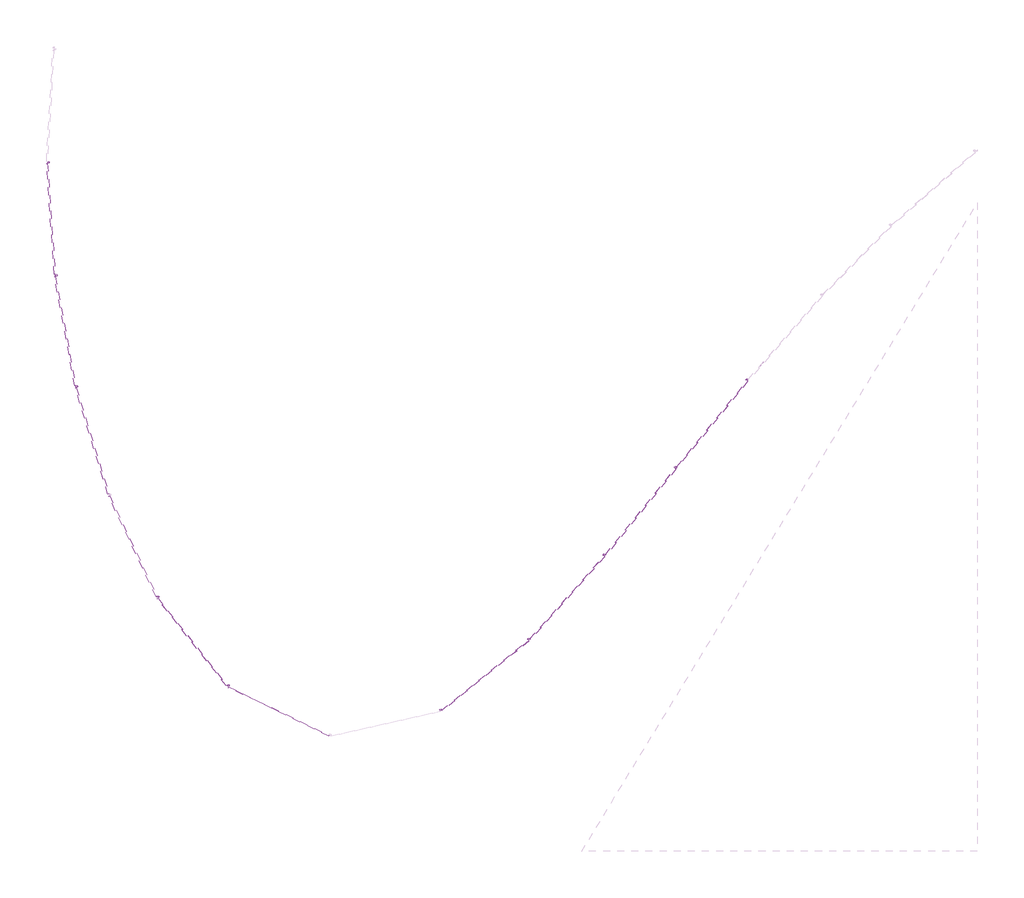
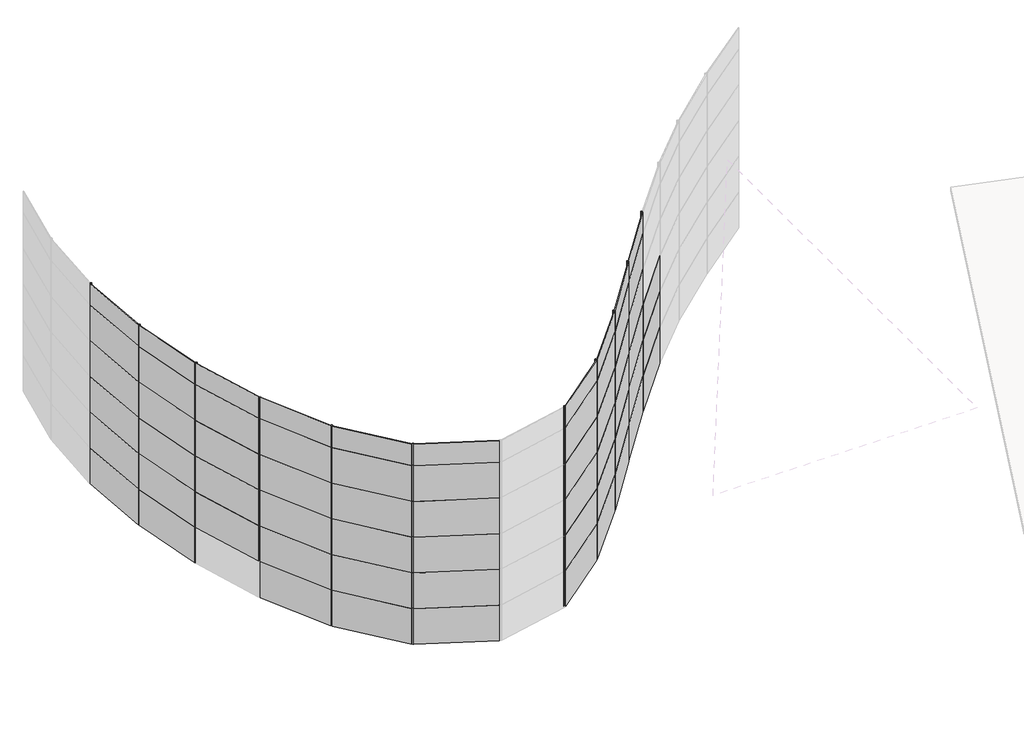
# One storey, part 4 of 8: 62 plates, 60 members.
"""IFC4 building model written with IfcOpenShell, lengths in millimetres."""

import ifcopenshell
import ifcopenshell.guid

model = None  # the IFC model being written
_history = None  # IfcOwnerHistory: only IFC2X3 demands one
_inside = {}  # id of a spatial element -> (the spatial element, [elements in it])
_under = {}  # id of a project, library or spatial element -> (it, [spatial elements below it])
_declared = {}  # id of a project -> (the project, [libraries it declares])
_typed = {}  # id of a type object -> (the type object, [elements of that type])
_made_of = {}  # id of a material, layer set ... -> (it, [elements and type objects made of it])


def new_model(schema):
    """Start an empty IFC model of exactly this schema.

    Asked for "IFC4X3", IfcOpenShell would pick the latest addendum, in which some entities
    have other attributes; the version numbers below select the first issue.
    IFC2X3 requires an IfcOwnerHistory on every rooted entity: one is made here for all.
    """
    global model, _history
    if schema == "IFC4X3":
        model = ifcopenshell.file(schema_version=(4, 3, 0, 0))
    else:
        model = ifcopenshell.file(schema=schema)
    _inside.clear()
    _under.clear()
    _declared.clear()
    _typed.clear()
    _made_of.clear()
    _history = None
    if model.schema == "IFC2X3":
        org = make("IfcOrganization", Name="unknown")
        user = make(
            "IfcPersonAndOrganization",
            ThePerson=make("IfcPerson", FamilyName="unknown"),
            TheOrganization=org,
        )
        app = make(
            "IfcApplication",
            ApplicationDeveloper=org,
            Version="unknown",
            ApplicationFullName="unknown",
            ApplicationIdentifier="unknown",
        )
        _history = make(
            "IfcOwnerHistory",
            OwningUser=user,
            OwningApplication=app,
            ChangeAction="ADDED",
            CreationDate=0,
        )
    return model


def make(cls, **values):
    """One entity of the class cls with the attributes given. An attribute that is None is left unset."""
    return model.create_entity(
        cls, **{name: value for name, value in values.items() if value is not None}
    )


def rooted(cls, **values):
    """An entity with a GlobalId (a new one), such as an element, a storey or a relation."""
    return make(cls, GlobalId=ifcopenshell.guid.new(), OwnerHistory=_history, **values)


def si_unit(unit_type, name, prefix=None):
    """IfcSIUnit, for example si_unit("LENGTHUNIT", "METRE", prefix="MILLI")."""
    return make("IfcSIUnit", UnitType=unit_type, Prefix=prefix, Name=name)


def assignment(units):
    """IfcUnitAssignment: the units of a project."""
    return None if units is None else make("IfcUnitAssignment", Units=units)


def point(xyz):
    """IfcCartesianPoint."""
    return None if xyz is None else make("IfcCartesianPoint", Coordinates=xyz)


def direction(xyz):
    """IfcDirection."""
    return None if xyz is None else make("IfcDirection", DirectionRatios=xyz)


def frame(location, z_axis=None, x_axis=None):
    """IfcAxis2Placement3D, a coordinate frame: its origin and axes. An axis left out is left unset."""
    return make(
        "IfcAxis2Placement3D",
        Location=point(location),
        Axis=direction(z_axis),
        RefDirection=direction(x_axis),
    )


def frame_2d(location, x_axis=None):
    """IfcAxis2Placement2D, a coordinate frame in the plane: its origin and x axis."""
    return make(
        "IfcAxis2Placement2D", Location=point(location), RefDirection=direction(x_axis)
    )


def origin():
    """The frame at (0, 0, 0) with its axes left unset."""
    return frame((0.0, 0.0, 0.0))


def origin_with_axes():
    """The frame at (0, 0, 0) with the z axis (0, 0, 1) and the x axis (1, 0, 0) written out."""
    return frame((0.0, 0.0, 0.0), z_axis=(0.0, 0.0, 1.0), x_axis=(1.0, 0.0, 0.0))


def origin_2d():
    """The frame at (0, 0) in the plane with its x axis left unset."""
    return frame_2d((0.0, 0.0))


def place(relative_to, where):
    """IfcLocalPlacement: puts the frame where relative to a parent placement (None: the world)."""
    return make(
        "IfcLocalPlacement", PlacementRelTo=relative_to, RelativePlacement=where
    )


def context(
    kind, dimensions, precision=None, world=None, true_north=None, identifier=None
):
    """IfcGeometricRepresentationContext, for example the 3D "Model" context."""
    return make(
        "IfcGeometricRepresentationContext",
        ContextIdentifier=identifier,
        ContextType=kind,
        CoordinateSpaceDimension=dimensions,
        Precision=precision,
        WorldCoordinateSystem=world,
        TrueNorth=true_north,
    )


def project(units=None, contexts=None):
    """IfcProject with its units and contexts."""
    return rooted(
        "IfcProject",
        Name="project",
        RepresentationContexts=contexts,
        UnitsInContext=assignment(units),
    )


def spatial(cls, under=None, at=None, **own):
    """A site, building, storey or space (cls), placed at a placement, below another one or the project."""
    s = rooted(cls, ObjectPlacement=at, **own)
    if under is not None:
        _under.setdefault(under.id(), (under, []))[1].append(s)
    return s


def polyline(points):
    """IfcPolyline through the points."""
    return make("IfcPolyline", Points=[point(p) for p in points])


def circle_curve(where, radius):
    """IfcCircle in the frame where."""
    return make("IfcCircle", Position=where, Radius=radius)


def trimmed(basis, trim1, trim2, sense, master):
    """IfcTrimmedCurve: the piece of a basis curve between two trims."""
    return make(
        "IfcTrimmedCurve",
        BasisCurve=basis,
        Trim1=trim1,
        Trim2=trim2,
        SenseAgreement=sense,
        MasterRepresentation=master,
    )


def segment(curve, same_sense, transition):
    """IfcCompositeCurveSegment."""
    return make(
        "IfcCompositeCurveSegment",
        Transition=transition,
        SameSense=same_sense,
        ParentCurve=curve,
    )


def composite_curve(segments, self_intersect=None):
    """IfcCompositeCurve: segments joined end to end."""
    return make("IfcCompositeCurve", Segments=segments, SelfIntersect=self_intersect)


def outline(outer, holes=None, kind="AREA"):
    """IfcArbitraryClosedProfileDef: a profile drawn as a closed curve; with holes, ...WithVoids."""
    if holes is None:
        return make("IfcArbitraryClosedProfileDef", ProfileType=kind, OuterCurve=outer)
    return make(
        "IfcArbitraryProfileDefWithVoids",
        ProfileType=kind,
        OuterCurve=outer,
        InnerCurves=holes,
    )


def extrude(swept, where, along, depth):
    """IfcExtrudedAreaSolid: the profile swept, set in the frame where, extruded along a direction by depth."""
    return make(
        "IfcExtrudedAreaSolid",
        SweptArea=swept,
        Position=where,
        ExtrudedDirection=direction(along),
        Depth=depth,
    )


def shape(context_of_items, identifier, shape_type, items):
    """IfcShapeRepresentation: the items that make up one representation, for example the "Body"."""
    return make(
        "IfcShapeRepresentation",
        ContextOfItems=context_of_items,
        RepresentationIdentifier=identifier,
        RepresentationType=shape_type,
        Items=items,
    )


def source(mapping_origin, context_of_items, identifier, shape_type, items):
    """IfcRepresentationMap: a shape defined once, which mapped items show again and again."""
    return make(
        "IfcRepresentationMap",
        MappingOrigin=mapping_origin,
        MappedRepresentation=shape(context_of_items, identifier, shape_type, items),
    )


def transform(
    local_origin,
    x_axis=None,
    y_axis=None,
    z_axis=None,
    scale=None,
    scale2=None,
    scale3=None,
    uniform=True,
):
    """IfcCartesianTransformationOperator3D, or its non-uniform kind. x_axis, y_axis, z_axis: its Axis1, 2, 3."""
    if uniform:
        return make(
            "IfcCartesianTransformationOperator3D",
            Axis1=direction(x_axis),
            Axis2=direction(y_axis),
            LocalOrigin=point(local_origin),
            Scale=scale,
            Axis3=direction(z_axis),
        )
    return make(
        "IfcCartesianTransformationOperator3DnonUniform",
        Axis1=direction(x_axis),
        Axis2=direction(y_axis),
        LocalOrigin=point(local_origin),
        Scale=scale,
        Axis3=direction(z_axis),
        Scale2=scale2,
        Scale3=scale3,
    )


def mapped(mapping_source, mapping_target):
    """IfcMappedItem: shows the shape of a source again, moved by a transform."""
    return make(
        "IfcMappedItem", MappingSource=mapping_source, MappingTarget=mapping_target
    )


def made_of(thing, what):
    """Note that an element or type object is made of a material, layer set ...; save() writes the relation."""
    if what is not None:
        _made_of.setdefault(what.id(), (what, []))[1].append(thing)
    return thing


def element(
    cls,
    number,
    at=None,
    inside=None,
    cuts=None,
    type_object=None,
    material=None,
    context=None,
    identifier="Body",
    shape_type=None,
    held_by="IfcProductDefinitionShape",
    body=None,
    shapes=None,
    **own,
):
    """One element of the class cls, such as IfcWall. Its Tag is "e" and its number.

    at: its placement. inside: the storey or other place that contains it. cuts: it is an
    opening in that element (IfcRelVoidsElement). A single representation is given by context,
    identifier, shape_type and body (its items); several are given by shapes. held_by: the class
    of the entity that holds the representations. save() writes the other relations.
    """
    e = rooted(cls, Tag="e%d" % number, ObjectPlacement=at, **own)
    if body is not None:
        shapes = [shape(context, identifier, shape_type, body)]
    if shapes is not None:
        e.Representation = make(held_by, Representations=shapes)
    if inside is not None:
        _inside.setdefault(inside.id(), (inside, []))[1].append(e)
    if cuts is not None:
        rooted(
            "IfcRelVoidsElement", RelatingBuildingElement=cuts, RelatedOpeningElement=e
        )
    if type_object is not None:
        _typed.setdefault(type_object.id(), (type_object, []))[1].append(e)
    return made_of(e, material)


def aggregate(whole, parts):
    """IfcRelAggregates: a whole, such as a stair, and the parts it consists of."""
    return rooted("IfcRelAggregates", RelatingObject=whole, RelatedObjects=parts)


def save(model, path):
    """Write the relations noted so far, then the file.

    IfcRelAggregates (storeys below a building ...), IfcRelContainedInSpatialStructure (elements
    in a storey), IfcRelDefinesByType, IfcRelAssociatesMaterial and IfcRelDeclares: one each for
    every whole, place, type object, material and project.
    """
    for whole, parts in _under.values():
        aggregate(whole, parts)
    for where, things in _inside.values():
        rooted(
            "IfcRelContainedInSpatialStructure",
            RelatedElements=things,
            RelatingStructure=where,
        )
    for kind, things in _typed.values():
        rooted("IfcRelDefinesByType", RelatedObjects=things, RelatingType=kind)
    for what, things in _made_of.values():
        rooted("IfcRelAssociatesMaterial", RelatedObjects=things, RelatingMaterial=what)
    for by, libraries in _declared.values():
        rooted("IfcRelDeclares", RelatingContext=by, RelatedDefinitions=libraries)
    model.write(path)


def montante_circular_25_mm_raio_36e581cf(model_context):
    return source(origin(), model_context, "Body", "SweptSolid", [
        extrude(outline(composite_curve([segment(trimmed(circle_curve(origin_2d(), 25.0), [point((25.0, 0.0))], [point((-25.0, 0.0))], False, "CARTESIAN"), True, "CONTINUOUS"), segment(trimmed(circle_curve(origin_2d(), 25.0), [point((-25.0, 0.0))], [point((25.0, 0.0))], False, "CARTESIAN"), True, "CONTINUOUS")], self_intersect=False)), frame((0.0, 0.0, -1500.0), z_axis=(0.0, 0.0, 1.0), x_axis=(1.0, 0.0, 0.0)), (0.0, 0.0, 1.0), 1500.0),
    ])


def montante_circular_25_mm_raio_8ba79aec(model_context):
    return source(origin(), model_context, "Body", "SweptSolid", [
        extrude(outline(composite_curve([segment(trimmed(circle_curve(origin_2d(), 25.0), [point((25.0, 0.0))], [point((-25.0, 0.0))], False, "CARTESIAN"), True, "CONTINUOUS"), segment(trimmed(circle_curve(origin_2d(), 25.0), [point((-25.0, 0.0))], [point((25.0, 0.0))], False, "CARTESIAN"), True, "CONTINUOUS")], self_intersect=False)), frame((0.0, 0.0, -900.0), z_axis=(0.0, 0.0, 1.0), x_axis=(1.0, 0.0, 0.0)), (0.0, 0.0, 1.0), 900.0),
    ])


def painel_do_sistema_85ccde5d(model_context):
    return source(origin(), model_context, "Body", "SweptSolid", [
        extrude(outline(polyline([(1475.0, -49.5), (-1475.0, -49.5), (-1475.0, -24.5), (1475.0, -24.5), (1475.0, -49.5)])), origin_with_axes(), (0.0, 0.0, 1.0), 1500.0),
    ])


def painel_do_sistema_d8fd150b(model_context):
    return source(origin(), model_context, "Body", "SweptSolid", [
        extrude(outline(polyline([(1475.0, -49.5), (-1475.0, -49.5), (-1475.0, -24.5), (1475.0, -24.5), (1475.0, -49.5)])), origin_with_axes(), (0.0, 0.0, 1.0), 900.0),
    ])


model = new_model("IFC4")

# Units and contexts
model_context = context("Model", 3, world=origin())
ifc_project = project(units=[si_unit("LENGTHUNIT", "METRE", prefix="MILLI")], contexts=[model_context])

# Site, building, storey
site = spatial("IfcSite", under=ifc_project)
building = spatial("IfcBuilding", under=site)
storey = spatial("IfcBuildingStorey", under=building, Name="Nível 3", Elevation=7695.2)

# Members
placement = place(None, origin())
montante_circular_25_mm_raio_shape = montante_circular_25_mm_raio_36e581cf(model_context)
element("IfcMember", 1, ObjectType="Montante circular : 25 mm Raio", at=placement, inside=storey, context=model_context, shape_type="MappedRepresentation", body=[
    mapped(montante_circular_25_mm_raio_shape, transform((-41927.7364355, 30807.566003, 9000.0), x_axis=(0.00926833746122375, -0.999957048037917, 0.0), y_axis=(-0.999957048037917, -0.00926833746122375, 0.0), z_axis=(0.0, 0.0, -1.0))),
])
element("IfcMember", 2, ObjectType="Montante circular : 25 mm Raio", at=placement, inside=storey, context=model_context, shape_type="MappedRepresentation", body=[
    mapped(montante_circular_25_mm_raio_shape, transform((-41719.5366875, 27814.7992454, 9000.0), x_axis=(0.12720739477424994, -0.9918761408133316, 0.0), y_axis=(-0.9918761408133316, -0.12720739477424994, 0.0), z_axis=(0.0, 0.0, -1.0))),
])
element("IfcMember", 3, ObjectType="Montante circular : 25 mm Raio", at=placement, inside=storey, context=model_context, shape_type="MappedRepresentation", body=[
    mapped(montante_circular_25_mm_raio_shape, transform((-41172.4912602, 24865.0973452, 9000.0), x_axis=(0.23687893376105146, -0.9715391761222125, 0.0), y_axis=(-0.9715391761222125, -0.23687893376105146, 0.0), z_axis=(0.0, 0.0, -1.0))),
])
element("IfcMember", 4, ObjectType="Montante circular : 25 mm Raio", at=placement, inside=storey, context=model_context, shape_type="MappedRepresentation", body=[
    mapped(montante_circular_25_mm_raio_shape, transform((-39014.8508906, 19282.6093761, 9000.0), x_axis=(0.5079873162147127, -0.8613645491689181, 0.0), y_axis=(-0.8613645491689181, -0.5079873162147127, 0.0), z_axis=(0.0, 0.0, -1.0))),
])
element("IfcMember", 5, ObjectType="Montante circular : 25 mm Raio", at=placement, inside=storey, context=model_context, shape_type="MappedRepresentation", body=[
    mapped(montante_circular_25_mm_raio_shape, transform((-37150.2365801, 16932.4575783, 9000.0), x_axis=(0.7466685294931728, -0.6651962921307538, 0.0), y_axis=(-0.6651962921307538, -0.7466685294931728, 0.0), z_axis=(0.0, 0.0, -1.0))),
])
element("IfcMember", 6, ObjectType="Montante circular : 25 mm Raio", at=placement, inside=storey, context=model_context, shape_type="MappedRepresentation", body=[
    mapped(montante_circular_25_mm_raio_shape, transform((-31525.1733328, 16282.9834173, 9000.0), x_axis=(0.870163483817595, 0.49276313927730647, 0.0), y_axis=(0.49276313927730647, -0.870163483817595, 0.0), z_axis=(0.0, 0.0, -1.0))),
])
element("IfcMember", 7, ObjectType="Montante circular : 25 mm Raio", at=placement, inside=storey, context=model_context, shape_type="MappedRepresentation", body=[
    mapped(montante_circular_25_mm_raio_shape, transform((-29189.3459235, 18165.5110569, 9000.0), x_axis=(0.7046961293095542, 0.7095092426009207, 0.0), y_axis=(0.7095092426009207, -0.7046961293095542, 0.0), z_axis=(0.0, 0.0, -1.0))),
])
element("IfcMember", 8, ObjectType="Montante circular : 25 mm Raio", at=placement, inside=storey, context=model_context, shape_type="MappedRepresentation", body=[
    mapped(montante_circular_25_mm_raio_shape, transform((-27187.2576877, 20399.7095029, 9000.0), x_axis=(0.6410206876840713, 0.7675236009146822, 0.0), y_axis=(0.7675236009146822, -0.6410206876840713, 0.0), z_axis=(0.0, 0.0, -1.0))),
])
element("IfcMember", 9, ObjectType="Montante circular : 25 mm Raio", at=placement, inside=storey, context=model_context, shape_type="MappedRepresentation", body=[
    mapped(montante_circular_25_mm_raio_shape, transform((-25293.7553869, 22726.6493467, 9000.0), x_axis=(0.627267192624168, 0.7788041275297628, 0.0), y_axis=(0.7788041275297628, -0.627267192624168, 0.0), z_axis=(0.0, 0.0, -1.0))),
])
element("IfcMember", 10, ObjectType="Montante circular : 25 mm Raio", at=placement, inside=storey, context=model_context, shape_type="MappedRepresentation", body=[
    mapped(montante_circular_25_mm_raio_shape, transform((-23394.8086307, 25049.1482632, 9000.0), x_axis=(0.6426798456549806, 0.766134854962813, 0.0), y_axis=(0.766134854962813, -0.6426798456549806, 0.0), z_axis=(0.0, 0.0, -1.0))),
])
element("IfcMember", 11, ObjectType="Montante circular : 25 mm Raio", at=placement, inside=storey, context=model_context, shape_type="MappedRepresentation", body=[
    mapped(montante_circular_25_mm_raio_shape, transform((-41927.7364355, 30807.566003, 10500.0), x_axis=(0.00926833746122375, -0.999957048037917, 0.0), y_axis=(-0.999957048037917, -0.00926833746122375, 0.0), z_axis=(0.0, 0.0, -1.0))),
])
element("IfcMember", 12, ObjectType="Montante circular : 25 mm Raio", at=placement, inside=storey, context=model_context, shape_type="MappedRepresentation", body=[
    mapped(montante_circular_25_mm_raio_shape, transform((-41719.5366875, 27814.7992454, 10500.0), x_axis=(0.12720739477424994, -0.9918761408133316, 0.0), y_axis=(-0.9918761408133316, -0.12720739477424994, 0.0), z_axis=(0.0, 0.0, -1.0))),
])
element("IfcMember", 13, ObjectType="Montante circular : 25 mm Raio", at=placement, inside=storey, context=model_context, shape_type="MappedRepresentation", body=[
    mapped(montante_circular_25_mm_raio_shape, transform((-41172.4912602, 24865.0973452, 10500.0), x_axis=(0.23687893376105146, -0.9715391761222125, 0.0), y_axis=(-0.9715391761222125, -0.23687893376105146, 0.0), z_axis=(0.0, 0.0, -1.0))),
])
element("IfcMember", 14, ObjectType="Montante circular : 25 mm Raio", at=placement, inside=storey, context=model_context, shape_type="MappedRepresentation", body=[
    mapped(montante_circular_25_mm_raio_shape, transform((-39014.8508906, 19282.6093761, 10500.0), x_axis=(0.5079873162147126, -0.8613645491689182, 0.0), y_axis=(-0.8613645491689182, -0.5079873162147126, 0.0), z_axis=(0.0, 0.0, -1.0))),
])
element("IfcMember", 15, ObjectType="Montante circular : 25 mm Raio", at=placement, inside=storey, context=model_context, shape_type="MappedRepresentation", body=[
    mapped(montante_circular_25_mm_raio_shape, transform((-37150.2365801, 16932.4575783, 10500.0), x_axis=(0.746668529493172, -0.6651962921307546, 0.0), y_axis=(-0.6651962921307546, -0.746668529493172, 0.0), z_axis=(0.0, 0.0, -1.0))),
])
element("IfcMember", 16, ObjectType="Montante circular : 25 mm Raio", at=placement, inside=storey, context=model_context, shape_type="MappedRepresentation", body=[
    mapped(montante_circular_25_mm_raio_shape, transform((-31525.1733328, 16282.9834173, 10500.0), x_axis=(0.870163483817595, 0.49276313927730647, 0.0), y_axis=(0.49276313927730647, -0.870163483817595, 0.0), z_axis=(0.0, 0.0, -1.0))),
])
element("IfcMember", 17, ObjectType="Montante circular : 25 mm Raio", at=placement, inside=storey, context=model_context, shape_type="MappedRepresentation", body=[
    mapped(montante_circular_25_mm_raio_shape, transform((-29189.3459235, 18165.5110569, 10500.0), x_axis=(0.7046961293095542, 0.7095092426009207, 0.0), y_axis=(0.7095092426009207, -0.7046961293095542, 0.0), z_axis=(0.0, 0.0, -1.0))),
])
element("IfcMember", 18, ObjectType="Montante circular : 25 mm Raio", at=placement, inside=storey, context=model_context, shape_type="MappedRepresentation", body=[
    mapped(montante_circular_25_mm_raio_shape, transform((-27187.2576877, 20399.7095029, 10500.0), x_axis=(0.6410206876840713, 0.7675236009146822, 0.0), y_axis=(0.7675236009146822, -0.6410206876840713, 0.0), z_axis=(0.0, 0.0, -1.0))),
])
element("IfcMember", 19, ObjectType="Montante circular : 25 mm Raio", at=placement, inside=storey, context=model_context, shape_type="MappedRepresentation", body=[
    mapped(montante_circular_25_mm_raio_shape, transform((-25293.7553869, 22726.6493467, 10500.0), x_axis=(0.627267192624168, 0.7788041275297628, 0.0), y_axis=(0.7788041275297628, -0.627267192624168, 0.0), z_axis=(0.0, 0.0, -1.0))),
])
element("IfcMember", 20, ObjectType="Montante circular : 25 mm Raio", at=placement, inside=storey, context=model_context, shape_type="MappedRepresentation", body=[
    mapped(montante_circular_25_mm_raio_shape, transform((-23394.8086307, 25049.1482632, 10500.0), x_axis=(0.6426798456549806, 0.766134854962813, 0.0), y_axis=(0.766134854962813, -0.6426798456549806, 0.0), z_axis=(0.0, 0.0, -1.0))),
])
element("IfcMember", 21, ObjectType="Montante circular : 25 mm Raio", at=placement, inside=storey, context=model_context, shape_type="MappedRepresentation", body=[
    mapped(montante_circular_25_mm_raio_shape, transform((-41927.7364355, 30807.566003, 12000.0), x_axis=(0.00926833746122375, -0.999957048037917, 0.0), y_axis=(-0.999957048037917, -0.00926833746122375, 0.0), z_axis=(0.0, 0.0, -1.0))),
])
element("IfcMember", 22, ObjectType="Montante circular : 25 mm Raio", at=placement, inside=storey, context=model_context, shape_type="MappedRepresentation", body=[
    mapped(montante_circular_25_mm_raio_shape, transform((-41719.5366875, 27814.7992454, 12000.0), x_axis=(0.12720739477424994, -0.9918761408133316, 0.0), y_axis=(-0.9918761408133316, -0.12720739477424994, 0.0), z_axis=(0.0, 0.0, -1.0))),
])
element("IfcMember", 23, ObjectType="Montante circular : 25 mm Raio", at=placement, inside=storey, context=model_context, shape_type="MappedRepresentation", body=[
    mapped(montante_circular_25_mm_raio_shape, transform((-41172.4912602, 24865.0973452, 12000.0), x_axis=(0.23687893376105146, -0.9715391761222125, 0.0), y_axis=(-0.9715391761222125, -0.23687893376105146, 0.0), z_axis=(0.0, 0.0, -1.0))),
])
element("IfcMember", 24, ObjectType="Montante circular : 25 mm Raio", at=placement, inside=storey, context=model_context, shape_type="MappedRepresentation", body=[
    mapped(montante_circular_25_mm_raio_shape, transform((-39014.8508906, 19282.6093761, 12000.0), x_axis=(0.5079873162147126, -0.8613645491689182, 0.0), y_axis=(-0.8613645491689182, -0.5079873162147126, 0.0), z_axis=(0.0, 0.0, -1.0))),
])
element("IfcMember", 25, ObjectType="Montante circular : 25 mm Raio", at=placement, inside=storey, context=model_context, shape_type="MappedRepresentation", body=[
    mapped(montante_circular_25_mm_raio_shape, transform((-37150.2365801, 16932.4575783, 12000.0), x_axis=(0.7466685294931724, -0.665196292130754, 0.0), y_axis=(-0.665196292130754, -0.7466685294931724, 0.0), z_axis=(0.0, 0.0, -1.0))),
])
element("IfcMember", 26, ObjectType="Montante circular : 25 mm Raio", at=placement, inside=storey, context=model_context, shape_type="MappedRepresentation", body=[
    mapped(montante_circular_25_mm_raio_shape, transform((-31525.1733328, 16282.9834173, 12000.0), x_axis=(0.870163483817595, 0.49276313927730647, 0.0), y_axis=(0.49276313927730647, -0.870163483817595, 0.0), z_axis=(0.0, 0.0, -1.0))),
])
element("IfcMember", 27, ObjectType="Montante circular : 25 mm Raio", at=placement, inside=storey, context=model_context, shape_type="MappedRepresentation", body=[
    mapped(montante_circular_25_mm_raio_shape, transform((-29189.3459235, 18165.5110569, 12000.0), x_axis=(0.7046961293095542, 0.7095092426009207, 0.0), y_axis=(0.7095092426009207, -0.7046961293095542, 0.0), z_axis=(0.0, 0.0, -1.0))),
])
element("IfcMember", 28, ObjectType="Montante circular : 25 mm Raio", at=placement, inside=storey, context=model_context, shape_type="MappedRepresentation", body=[
    mapped(montante_circular_25_mm_raio_shape, transform((-27187.2576877, 20399.7095029, 12000.0), x_axis=(0.6410206876840713, 0.7675236009146822, 0.0), y_axis=(0.7675236009146822, -0.6410206876840713, 0.0), z_axis=(0.0, 0.0, -1.0))),
])
element("IfcMember", 29, ObjectType="Montante circular : 25 mm Raio", at=placement, inside=storey, context=model_context, shape_type="MappedRepresentation", body=[
    mapped(montante_circular_25_mm_raio_shape, transform((-25293.7553869, 22726.6493467, 12000.0), x_axis=(0.627267192624168, 0.7788041275297628, 0.0), y_axis=(0.7788041275297628, -0.627267192624168, 0.0), z_axis=(0.0, 0.0, -1.0))),
])
element("IfcMember", 30, ObjectType="Montante circular : 25 mm Raio", at=placement, inside=storey, context=model_context, shape_type="MappedRepresentation", body=[
    mapped(montante_circular_25_mm_raio_shape, transform((-23394.8086307, 25049.1482632, 12000.0), x_axis=(0.6426798456549806, 0.766134854962813, 0.0), y_axis=(0.766134854962813, -0.6426798456549806, 0.0), z_axis=(0.0, 0.0, -1.0))),
])
element("IfcMember", 31, ObjectType="Montante circular : 25 mm Raio", at=placement, inside=storey, context=model_context, shape_type="MappedRepresentation", body=[
    mapped(montante_circular_25_mm_raio_shape, transform((-41927.7364355, 30807.566003, 13500.0), x_axis=(0.00926833746122375, -0.999957048037917, 0.0), y_axis=(-0.999957048037917, -0.00926833746122375, 0.0), z_axis=(0.0, 0.0, -1.0))),
])
element("IfcMember", 32, ObjectType="Montante circular : 25 mm Raio", at=placement, inside=storey, context=model_context, shape_type="MappedRepresentation", body=[
    mapped(montante_circular_25_mm_raio_shape, transform((-41719.5366875, 27814.7992454, 13500.0), x_axis=(0.12720739477424994, -0.9918761408133316, 0.0), y_axis=(-0.9918761408133316, -0.12720739477424994, 0.0), z_axis=(0.0, 0.0, -1.0))),
])
element("IfcMember", 33, ObjectType="Montante circular : 25 mm Raio", at=placement, inside=storey, context=model_context, shape_type="MappedRepresentation", body=[
    mapped(montante_circular_25_mm_raio_shape, transform((-41172.4912602, 24865.0973452, 13500.0), x_axis=(0.23687893376105146, -0.9715391761222125, 0.0), y_axis=(-0.9715391761222125, -0.23687893376105146, 0.0), z_axis=(0.0, 0.0, -1.0))),
])
element("IfcMember", 34, ObjectType="Montante circular : 25 mm Raio", at=placement, inside=storey, context=model_context, shape_type="MappedRepresentation", body=[
    mapped(montante_circular_25_mm_raio_shape, transform((-39014.8508906, 19282.6093761, 13500.0), x_axis=(0.5079873162147124, -0.8613645491689182, 0.0), y_axis=(-0.8613645491689182, -0.5079873162147124, 0.0), z_axis=(0.0, 0.0, -1.0))),
])
element("IfcMember", 35, ObjectType="Montante circular : 25 mm Raio", at=placement, inside=storey, context=model_context, shape_type="MappedRepresentation", body=[
    mapped(montante_circular_25_mm_raio_shape, transform((-37150.2365801, 16932.4575783, 13500.0), x_axis=(0.7466685294931728, -0.6651962921307538, 0.0), y_axis=(-0.6651962921307538, -0.7466685294931728, 0.0), z_axis=(0.0, 0.0, -1.0))),
])
element("IfcMember", 36, ObjectType="Montante circular : 25 mm Raio", at=placement, inside=storey, context=model_context, shape_type="MappedRepresentation", body=[
    mapped(montante_circular_25_mm_raio_shape, transform((-31525.1733328, 16282.9834173, 13500.0), x_axis=(0.870163483817595, 0.49276313927730647, 0.0), y_axis=(0.49276313927730647, -0.870163483817595, 0.0), z_axis=(0.0, 0.0, -1.0))),
])
element("IfcMember", 37, ObjectType="Montante circular : 25 mm Raio", at=placement, inside=storey, context=model_context, shape_type="MappedRepresentation", body=[
    mapped(montante_circular_25_mm_raio_shape, transform((-29189.3459235, 18165.5110569, 13500.0), x_axis=(0.7046961293095542, 0.7095092426009207, 0.0), y_axis=(0.7095092426009207, -0.7046961293095542, 0.0), z_axis=(0.0, 0.0, -1.0))),
])
element("IfcMember", 38, ObjectType="Montante circular : 25 mm Raio", at=placement, inside=storey, context=model_context, shape_type="MappedRepresentation", body=[
    mapped(montante_circular_25_mm_raio_shape, transform((-27187.2576877, 20399.7095029, 13500.0), x_axis=(0.6410206876840709, 0.7675236009146824, 0.0), y_axis=(0.7675236009146824, -0.6410206876840709, 0.0), z_axis=(0.0, 0.0, -1.0))),
])
element("IfcMember", 39, ObjectType="Montante circular : 25 mm Raio", at=placement, inside=storey, context=model_context, shape_type="MappedRepresentation", body=[
    mapped(montante_circular_25_mm_raio_shape, transform((-25293.7553869, 22726.6493467, 13500.0), x_axis=(0.627267192624168, 0.7788041275297628, 0.0), y_axis=(0.7788041275297628, -0.627267192624168, 0.0), z_axis=(0.0, 0.0, -1.0))),
])
element("IfcMember", 40, ObjectType="Montante circular : 25 mm Raio", at=placement, inside=storey, context=model_context, shape_type="MappedRepresentation", body=[
    mapped(montante_circular_25_mm_raio_shape, transform((-23394.8086307, 25049.1482632, 13500.0), x_axis=(0.6426798456549806, 0.766134854962813, 0.0), y_axis=(0.766134854962813, -0.6426798456549806, 0.0), z_axis=(0.0, 0.0, -1.0))),
])
element("IfcMember", 41, ObjectType="Montante circular : 25 mm Raio", at=placement, inside=storey, context=model_context, shape_type="MappedRepresentation", body=[
    mapped(montante_circular_25_mm_raio_shape, transform((-41927.7364355, 30807.566003, 15000.0), x_axis=(0.00926833746122375, -0.999957048037917, 0.0), y_axis=(-0.999957048037917, -0.00926833746122375, 0.0), z_axis=(0.0, 0.0, -1.0))),
])
element("IfcMember", 42, ObjectType="Montante circular : 25 mm Raio", at=placement, inside=storey, context=model_context, shape_type="MappedRepresentation", body=[
    mapped(montante_circular_25_mm_raio_shape, transform((-41719.5366875, 27814.7992454, 15000.0), x_axis=(0.12720739477424994, -0.9918761408133316, 0.0), y_axis=(-0.9918761408133316, -0.12720739477424994, 0.0), z_axis=(0.0, 0.0, -1.0))),
])
element("IfcMember", 43, ObjectType="Montante circular : 25 mm Raio", at=placement, inside=storey, context=model_context, shape_type="MappedRepresentation", body=[
    mapped(montante_circular_25_mm_raio_shape, transform((-41172.4912602, 24865.0973452, 15000.0), x_axis=(0.23687893376105146, -0.9715391761222125, 0.0), y_axis=(-0.9715391761222125, -0.23687893376105146, 0.0), z_axis=(0.0, 0.0, -1.0))),
])
element("IfcMember", 44, ObjectType="Montante circular : 25 mm Raio", at=placement, inside=storey, context=model_context, shape_type="MappedRepresentation", body=[
    mapped(montante_circular_25_mm_raio_shape, transform((-39014.8508906, 19282.6093761, 15000.0), x_axis=(0.5079873162147126, -0.8613645491689182, 0.0), y_axis=(-0.8613645491689182, -0.5079873162147126, 0.0), z_axis=(0.0, 0.0, -1.0))),
])
element("IfcMember", 45, ObjectType="Montante circular : 25 mm Raio", at=placement, inside=storey, context=model_context, shape_type="MappedRepresentation", body=[
    mapped(montante_circular_25_mm_raio_shape, transform((-37150.2365801, 16932.4575783, 15000.0), x_axis=(0.7466685294931728, -0.6651962921307538, 0.0), y_axis=(-0.6651962921307538, -0.7466685294931728, 0.0), z_axis=(0.0, 0.0, -1.0))),
])
element("IfcMember", 46, ObjectType="Montante circular : 25 mm Raio", at=placement, inside=storey, context=model_context, shape_type="MappedRepresentation", body=[
    mapped(montante_circular_25_mm_raio_shape, transform((-31525.1733328, 16282.9834173, 15000.0), x_axis=(0.870163483817595, 0.49276313927730647, 0.0), y_axis=(0.49276313927730647, -0.870163483817595, 0.0), z_axis=(0.0, 0.0, -1.0))),
])
element("IfcMember", 47, ObjectType="Montante circular : 25 mm Raio", at=placement, inside=storey, context=model_context, shape_type="MappedRepresentation", body=[
    mapped(montante_circular_25_mm_raio_shape, transform((-29189.3459235, 18165.5110569, 15000.0), x_axis=(0.7046961293095542, 0.7095092426009207, 0.0), y_axis=(0.7095092426009207, -0.7046961293095542, 0.0), z_axis=(0.0, 0.0, -1.0))),
])
element("IfcMember", 48, ObjectType="Montante circular : 25 mm Raio", at=placement, inside=storey, context=model_context, shape_type="MappedRepresentation", body=[
    mapped(montante_circular_25_mm_raio_shape, transform((-27187.2576877, 20399.7095029, 15000.0), x_axis=(0.6410206876840713, 0.7675236009146822, 0.0), y_axis=(0.7675236009146822, -0.6410206876840713, 0.0), z_axis=(0.0, 0.0, -1.0))),
])
element("IfcMember", 49, ObjectType="Montante circular : 25 mm Raio", at=placement, inside=storey, context=model_context, shape_type="MappedRepresentation", body=[
    mapped(montante_circular_25_mm_raio_shape, transform((-25293.7553869, 22726.6493467, 15000.0), x_axis=(0.627267192624168, 0.7788041275297628, 0.0), y_axis=(0.7788041275297628, -0.627267192624168, 0.0), z_axis=(0.0, 0.0, -1.0))),
])
element("IfcMember", 50, ObjectType="Montante circular : 25 mm Raio", at=placement, inside=storey, context=model_context, shape_type="MappedRepresentation", body=[
    mapped(montante_circular_25_mm_raio_shape, transform((-23394.8086307, 25049.1482632, 15000.0), x_axis=(0.6426798456549805, 0.7661348549628131, 0.0), y_axis=(0.7661348549628131, -0.6426798456549805, 0.0), z_axis=(0.0, 0.0, -1.0))),
])
montante_circular_25_mm_raio_2_shape = montante_circular_25_mm_raio_8ba79aec(model_context)
element("IfcMember", 51, ObjectType="Montante circular : 25 mm Raio", at=placement, inside=storey, context=model_context, shape_type="MappedRepresentation", body=[
    mapped(montante_circular_25_mm_raio_2_shape, transform((-41927.7364355, 30807.566003, 16500.0), x_axis=(0.00926833746122375, -0.999957048037917, 0.0), y_axis=(-0.999957048037917, -0.00926833746122375, 0.0), z_axis=(0.0, 0.0, -1.0))),
])
element("IfcMember", 52, ObjectType="Montante circular : 25 mm Raio", at=placement, inside=storey, context=model_context, shape_type="MappedRepresentation", body=[
    mapped(montante_circular_25_mm_raio_2_shape, transform((-41719.5366875, 27814.7992454, 16500.0), x_axis=(0.12720739477424994, -0.9918761408133316, 0.0), y_axis=(-0.9918761408133316, -0.12720739477424994, 0.0), z_axis=(0.0, 0.0, -1.0))),
])
element("IfcMember", 53, ObjectType="Montante circular : 25 mm Raio", at=placement, inside=storey, context=model_context, shape_type="MappedRepresentation", body=[
    mapped(montante_circular_25_mm_raio_2_shape, transform((-41172.4912602, 24865.0973452, 16500.0), x_axis=(0.23687893376105146, -0.9715391761222125, 0.0), y_axis=(-0.9715391761222125, -0.23687893376105146, 0.0), z_axis=(0.0, 0.0, -1.0))),
])
element("IfcMember", 54, ObjectType="Montante circular : 25 mm Raio", at=placement, inside=storey, context=model_context, shape_type="MappedRepresentation", body=[
    mapped(montante_circular_25_mm_raio_2_shape, transform((-39014.8508906, 19282.6093761, 16500.0), x_axis=(0.5079873162147126, -0.8613645491689182, 0.0), y_axis=(-0.8613645491689182, -0.5079873162147126, 0.0), z_axis=(0.0, 0.0, -1.0))),
])
element("IfcMember", 55, ObjectType="Montante circular : 25 mm Raio", at=placement, inside=storey, context=model_context, shape_type="MappedRepresentation", body=[
    mapped(montante_circular_25_mm_raio_2_shape, transform((-37150.2365801, 16932.4575783, 16500.0), x_axis=(0.7466685294931728, -0.6651962921307538, 0.0), y_axis=(-0.6651962921307538, -0.7466685294931728, 0.0), z_axis=(0.0, 0.0, -1.0))),
])
element("IfcMember", 56, ObjectType="Montante circular : 25 mm Raio", at=placement, inside=storey, context=model_context, shape_type="MappedRepresentation", body=[
    mapped(montante_circular_25_mm_raio_2_shape, transform((-31525.1733328, 16282.9834173, 16500.0), x_axis=(0.870163483817595, 0.49276313927730647, 0.0), y_axis=(0.49276313927730647, -0.870163483817595, 0.0), z_axis=(0.0, 0.0, -1.0))),
])
element("IfcMember", 57, ObjectType="Montante circular : 25 mm Raio", at=placement, inside=storey, context=model_context, shape_type="MappedRepresentation", body=[
    mapped(montante_circular_25_mm_raio_2_shape, transform((-29189.3459235, 18165.5110569, 16500.0), x_axis=(0.7046961293095542, 0.7095092426009207, 0.0), y_axis=(0.7095092426009207, -0.7046961293095542, 0.0), z_axis=(0.0, 0.0, -1.0))),
])
element("IfcMember", 58, ObjectType="Montante circular : 25 mm Raio", at=placement, inside=storey, context=model_context, shape_type="MappedRepresentation", body=[
    mapped(montante_circular_25_mm_raio_2_shape, transform((-27187.2576877, 20399.7095029, 16500.0), x_axis=(0.6410206876840713, 0.7675236009146822, 0.0), y_axis=(0.7675236009146822, -0.6410206876840713, 0.0), z_axis=(0.0, 0.0, -1.0))),
])
element("IfcMember", 59, ObjectType="Montante circular : 25 mm Raio", at=placement, inside=storey, context=model_context, shape_type="MappedRepresentation", body=[
    mapped(montante_circular_25_mm_raio_2_shape, transform((-25293.7553869, 22726.6493467, 16500.0), x_axis=(0.627267192624168, 0.7788041275297628, 0.0), y_axis=(0.7788041275297628, -0.627267192624168, 0.0), z_axis=(0.0, 0.0, -1.0))),
])
element("IfcMember", 60, ObjectType="Montante circular : 25 mm Raio", at=placement, inside=storey, context=model_context, shape_type="MappedRepresentation", body=[
    mapped(montante_circular_25_mm_raio_2_shape, transform((-23394.8086307, 25049.1482632, 16500.0), x_axis=(0.6426798456549805, 0.766134854962813, 0.0), y_axis=(0.766134854962813, -0.6426798456549805, 0.0), z_axis=(0.0, 0.0, -1.0))),
])

# Plates
painel_do_sistema_shape = painel_do_sistema_85ccde5d(model_context)
element("IfcPlate", 61, ObjectType="Painel do sistema : Envidraçado", at=placement, inside=storey, context=model_context, shape_type="MappedRepresentation", body=[
    mapped(painel_do_sistema_shape, transform((-41823.6365615, 29311.1826242, 9000.0), x_axis=(0.06939991602576077, -0.9975889191724302, 0.0), y_axis=(0.9975889191724302, 0.06939991602576077, 0.0), z_axis=(0.0, 0.0, 1.0))),
])
element("IfcPlate", 62, ObjectType="Painel do sistema : Envidraçado", at=placement, inside=storey, context=model_context, shape_type="MappedRepresentation", body=[
    mapped(painel_do_sistema_shape, transform((-41446.0139738, 26339.9482953, 9000.0), x_axis=(0.18234847575688512, -0.9832339667592555, 0.0), y_axis=(0.9832339667592555, 0.18234847575688512, 0.0), z_axis=(0.0, 0.0, 1.0))),
])
element("IfcPlate", 63, ObjectType="Painel do sistema : Envidraçado", at=placement, inside=storey, context=model_context, shape_type="MappedRepresentation", body=[
    mapped(painel_do_sistema_shape, transform((-39653.3088654, 20639.9492062, 9000.0), x_axis=(0.4256386498833567, -0.9048932200682429, 0.0), y_axis=(0.9048932200682429, 0.4256386498833567, 0.0), z_axis=(0.0, 0.0, 1.0))),
])
element("IfcPlate", 64, ObjectType="Painel do sistema : Envidraçado", at=placement, inside=storey, context=model_context, shape_type="MappedRepresentation", body=[
    mapped(painel_do_sistema_shape, transform((-38082.5437353, 18107.5334772, 9000.0), x_axis=(0.6215381034984806, -0.7833839326278731, 0.0), y_axis=(0.7833839326278731, 0.6215381034984806, 0.0), z_axis=(0.0, 0.0, 1.0))),
])
element("IfcPlate", 65, ObjectType="Painel do sistema : Envidraçado", at=placement, inside=storey, context=model_context, shape_type="MappedRepresentation", body=[
    mapped(painel_do_sistema_shape, transform((-35800.8656275, 16277.3255058, 9000.0), x_axis=(0.8995806350580464, -0.4367547149471449, 0.0), y_axis=(0.4367547149471449, 0.8995806350580464, 0.0), z_axis=(0.0, 0.0, 1.0))),
])
element("IfcPlate", 66, ObjectType="Painel do sistema : Envidraçado", at=placement, inside=storey, context=model_context, shape_type="MappedRepresentation", body=[
    mapped(painel_do_sistema_shape, transform((-30357.2596282, 17224.2472371, 9000.0), x_axis=(0.7786091364439218, 0.6275092131961494, 0.0), y_axis=(-0.6275092131961494, 0.7786091364439218, 0.0), z_axis=(0.0, 0.0, 1.0))),
])
element("IfcPlate", 67, ObjectType="Painel do sistema : Envidraçado", at=placement, inside=storey, context=model_context, shape_type="MappedRepresentation", body=[
    mapped(painel_do_sistema_shape, transform((-28188.3018056, 19282.6102799, 9000.0), x_axis=(0.6673627452593464, 0.7447328153370905, 0.0), y_axis=(-0.7447328153370905, 0.6673627452593464, 0.0), z_axis=(0.0, 0.0, 1.0))),
])
element("IfcPlate", 68, ObjectType="Painel do sistema : Envidraçado", at=placement, inside=storey, context=model_context, shape_type="MappedRepresentation", body=[
    mapped(painel_do_sistema_shape, transform((-26240.5065373, 21563.1794248, 9000.0), x_axis=(0.631167433620949, 0.7756466145973597, 0.0), y_axis=(-0.7756466145973597, 0.631167433620949, 0.0), z_axis=(0.0, 0.0, 1.0))),
])
element("IfcPlate", 69, ObjectType="Painel do sistema : Envidraçado", at=placement, inside=storey, context=model_context, shape_type="MappedRepresentation", body=[
    mapped(painel_do_sistema_shape, transform((-24344.2820088, 23887.898805, 9000.0), x_axis=(0.6329822520721655, 0.7741663054936256, 0.0), y_axis=(-0.7741663054936256, 0.6329822520721655, 0.0), z_axis=(0.0, 0.0, 1.0))),
])
element("IfcPlate", 70, ObjectType="Painel do sistema : Envidraçado", at=placement, inside=storey, context=model_context, shape_type="MappedRepresentation", body=[
    mapped(painel_do_sistema_shape, transform((-22405.4534016, 26176.6127774, 9000.0), x_axis=(0.6595701527276366, 0.751643009433895, 0.0), y_axis=(-0.751643009433895, 0.6595701527276366, 0.0), z_axis=(0.0, 0.0, 1.0))),
])
element("IfcPlate", 71, ObjectType="Painel do sistema : Envidraçado", at=placement, inside=storey, context=model_context, shape_type="MappedRepresentation", body=[
    mapped(painel_do_sistema_shape, transform((-41823.6365615, 29311.1826242, 10500.0), x_axis=(0.06939991602576077, -0.9975889191724302, 0.0), y_axis=(0.9975889191724302, 0.06939991602576077, 0.0), z_axis=(0.0, 0.0, 1.0))),
])
element("IfcPlate", 72, ObjectType="Painel do sistema : Envidraçado", at=placement, inside=storey, context=model_context, shape_type="MappedRepresentation", body=[
    mapped(painel_do_sistema_shape, transform((-41446.0139738, 26339.9482953, 10500.0), x_axis=(0.18234847575688515, -0.9832339667592555, 0.0), y_axis=(0.9832339667592555, 0.18234847575688515, 0.0), z_axis=(0.0, 0.0, 1.0))),
])
element("IfcPlate", 73, ObjectType="Painel do sistema : Envidraçado", at=placement, inside=storey, context=model_context, shape_type="MappedRepresentation", body=[
    mapped(painel_do_sistema_shape, transform((-40732.1290502, 23431.1931908, 10500.0), x_axis=(0.29357480664789803, -0.9559361029387107, 0.0), y_axis=(0.9559361029387107, 0.29357480664789803, 0.0), z_axis=(0.0, 0.0, 1.0))),
])
element("IfcPlate", 74, ObjectType="Painel do sistema : Envidraçado", at=placement, inside=storey, context=model_context, shape_type="MappedRepresentation", body=[
    mapped(painel_do_sistema_shape, transform((-39653.3088654, 20639.9492062, 10500.0), x_axis=(0.42563864988335665, -0.9048932200682429, 0.0), y_axis=(0.9048932200682429, 0.42563864988335665, 0.0), z_axis=(0.0, 0.0, 1.0))),
])
element("IfcPlate", 75, ObjectType="Painel do sistema : Envidraçado", at=placement, inside=storey, context=model_context, shape_type="MappedRepresentation", body=[
    mapped(painel_do_sistema_shape, transform((-38082.5437353, 18107.5334772, 10500.0), x_axis=(0.6215381034984807, -0.7833839326278731, 0.0), y_axis=(0.7833839326278731, 0.6215381034984807, 0.0), z_axis=(0.0, 0.0, 1.0))),
])
element("IfcPlate", 76, ObjectType="Painel do sistema : Envidraçado", at=placement, inside=storey, context=model_context, shape_type="MappedRepresentation", body=[
    mapped(painel_do_sistema_shape, transform((-35800.8656275, 16277.3255058, 10500.0), x_axis=(0.8995806350580465, -0.4367547149471449, 0.0), y_axis=(0.4367547149471449, 0.8995806350580465, 0.0), z_axis=(0.0, 0.0, 1.0))),
])
element("IfcPlate", 77, ObjectType="Painel do sistema : Envidraçado", at=placement, inside=storey, context=model_context, shape_type="MappedRepresentation", body=[
    mapped(painel_do_sistema_shape, transform((-30357.2596282, 17224.2472371, 10500.0), x_axis=(0.7786091364439218, 0.6275092131961494, 0.0), y_axis=(-0.6275092131961494, 0.7786091364439218, 0.0), z_axis=(0.0, 0.0, 1.0))),
])
element("IfcPlate", 78, ObjectType="Painel do sistema : Envidraçado", at=placement, inside=storey, context=model_context, shape_type="MappedRepresentation", body=[
    mapped(painel_do_sistema_shape, transform((-28188.3018056, 19282.6102799, 10500.0), x_axis=(0.6673627452593465, 0.7447328153370903, 0.0), y_axis=(-0.7447328153370903, 0.6673627452593465, 0.0), z_axis=(0.0, 0.0, 1.0))),
])
element("IfcPlate", 79, ObjectType="Painel do sistema : Envidraçado", at=placement, inside=storey, context=model_context, shape_type="MappedRepresentation", body=[
    mapped(painel_do_sistema_shape, transform((-26240.5065373, 21563.1794248, 10500.0), x_axis=(0.631167433620949, 0.7756466145973597, 0.0), y_axis=(-0.7756466145973597, 0.631167433620949, 0.0), z_axis=(0.0, 0.0, 1.0))),
])
element("IfcPlate", 80, ObjectType="Painel do sistema : Envidraçado", at=placement, inside=storey, context=model_context, shape_type="MappedRepresentation", body=[
    mapped(painel_do_sistema_shape, transform((-24344.2820088, 23887.898805, 10500.0), x_axis=(0.6329822520721655, 0.7741663054936256, 0.0), y_axis=(-0.7741663054936256, 0.6329822520721655, 0.0), z_axis=(0.0, 0.0, 1.0))),
])
element("IfcPlate", 81, ObjectType="Painel do sistema : Envidraçado", at=placement, inside=storey, context=model_context, shape_type="MappedRepresentation", body=[
    mapped(painel_do_sistema_shape, transform((-22405.4534016, 26176.6127774, 10500.0), x_axis=(0.6595701527276365, 0.7516430094338951, 0.0), y_axis=(-0.7516430094338951, 0.6595701527276365, 0.0), z_axis=(0.0, 0.0, 1.0))),
])
element("IfcPlate", 82, ObjectType="Painel do sistema : Envidraçado", at=placement, inside=storey, context=model_context, shape_type="MappedRepresentation", body=[
    mapped(painel_do_sistema_shape, transform((-41823.6365615, 29311.1826242, 12000.0), x_axis=(0.06939991602576077, -0.9975889191724302, 0.0), y_axis=(0.9975889191724302, 0.06939991602576077, 0.0), z_axis=(0.0, 0.0, 1.0))),
])
element("IfcPlate", 83, ObjectType="Painel do sistema : Envidraçado", at=placement, inside=storey, context=model_context, shape_type="MappedRepresentation", body=[
    mapped(painel_do_sistema_shape, transform((-41446.0139738, 26339.9482953, 12000.0), x_axis=(0.18234847575688515, -0.9832339667592555, 0.0), y_axis=(0.9832339667592555, 0.18234847575688515, 0.0), z_axis=(0.0, 0.0, 1.0))),
])
element("IfcPlate", 84, ObjectType="Painel do sistema : Envidraçado", at=placement, inside=storey, context=model_context, shape_type="MappedRepresentation", body=[
    mapped(painel_do_sistema_shape, transform((-40732.1290502, 23431.1931908, 12000.0), x_axis=(0.29357480664789803, -0.9559361029387107, 0.0), y_axis=(0.9559361029387107, 0.29357480664789803, 0.0), z_axis=(0.0, 0.0, 1.0))),
])
element("IfcPlate", 85, ObjectType="Painel do sistema : Envidraçado", at=placement, inside=storey, context=model_context, shape_type="MappedRepresentation", body=[
    mapped(painel_do_sistema_shape, transform((-39653.3088654, 20639.9492062, 12000.0), x_axis=(0.42563864988335665, -0.9048932200682429, 0.0), y_axis=(0.9048932200682429, 0.42563864988335665, 0.0), z_axis=(0.0, 0.0, 1.0))),
])
element("IfcPlate", 86, ObjectType="Painel do sistema : Envidraçado", at=placement, inside=storey, context=model_context, shape_type="MappedRepresentation", body=[
    mapped(painel_do_sistema_shape, transform((-38082.5437353, 18107.5334772, 12000.0), x_axis=(0.6215381034984816, -0.7833839326278723, 0.0), y_axis=(0.7833839326278723, 0.6215381034984816, 0.0), z_axis=(0.0, 0.0, 1.0))),
])
element("IfcPlate", 87, ObjectType="Painel do sistema : Envidraçado", at=placement, inside=storey, context=model_context, shape_type="MappedRepresentation", body=[
    mapped(painel_do_sistema_shape, transform((-35800.8656275, 16277.3255058, 12000.0), x_axis=(0.8995806350580463, -0.4367547149471455, 0.0), y_axis=(0.4367547149471455, 0.8995806350580463, 0.0), z_axis=(0.0, 0.0, 1.0))),
])
element("IfcPlate", 88, ObjectType="Painel do sistema : Envidraçado", at=placement, inside=storey, context=model_context, shape_type="MappedRepresentation", body=[
    mapped(painel_do_sistema_shape, transform((-30357.2596282, 17224.2472371, 12000.0), x_axis=(0.7786091364439218, 0.6275092131961494, 0.0), y_axis=(-0.6275092131961494, 0.7786091364439218, 0.0), z_axis=(0.0, 0.0, 1.0))),
])
element("IfcPlate", 89, ObjectType="Painel do sistema : Envidraçado", at=placement, inside=storey, context=model_context, shape_type="MappedRepresentation", body=[
    mapped(painel_do_sistema_shape, transform((-28188.3018056, 19282.6102799, 12000.0), x_axis=(0.6673627452593465, 0.7447328153370903, 0.0), y_axis=(-0.7447328153370903, 0.6673627452593465, 0.0), z_axis=(0.0, 0.0, 1.0))),
])
element("IfcPlate", 90, ObjectType="Painel do sistema : Envidraçado", at=placement, inside=storey, context=model_context, shape_type="MappedRepresentation", body=[
    mapped(painel_do_sistema_shape, transform((-26240.5065373, 21563.1794248, 12000.0), x_axis=(0.631167433620949, 0.7756466145973597, 0.0), y_axis=(-0.7756466145973597, 0.631167433620949, 0.0), z_axis=(0.0, 0.0, 1.0))),
])
element("IfcPlate", 91, ObjectType="Painel do sistema : Envidraçado", at=placement, inside=storey, context=model_context, shape_type="MappedRepresentation", body=[
    mapped(painel_do_sistema_shape, transform((-24344.2820088, 23887.898805, 12000.0), x_axis=(0.6329822520721655, 0.7741663054936256, 0.0), y_axis=(-0.7741663054936256, 0.6329822520721655, 0.0), z_axis=(0.0, 0.0, 1.0))),
])
element("IfcPlate", 92, ObjectType="Painel do sistema : Envidraçado", at=placement, inside=storey, context=model_context, shape_type="MappedRepresentation", body=[
    mapped(painel_do_sistema_shape, transform((-22405.4534016, 26176.6127774, 12000.0), x_axis=(0.6595701527276365, 0.7516430094338951, 0.0), y_axis=(-0.7516430094338951, 0.6595701527276365, 0.0), z_axis=(0.0, 0.0, 1.0))),
])
element("IfcPlate", 93, ObjectType="Painel do sistema : Envidraçado", at=placement, inside=storey, context=model_context, shape_type="MappedRepresentation", body=[
    mapped(painel_do_sistema_shape, transform((-41823.6365615, 29311.1826242, 13500.0), x_axis=(0.06939991602576077, -0.9975889191724302, 0.0), y_axis=(0.9975889191724302, 0.06939991602576077, 0.0), z_axis=(0.0, 0.0, 1.0))),
])
element("IfcPlate", 94, ObjectType="Painel do sistema : Envidraçado", at=placement, inside=storey, context=model_context, shape_type="MappedRepresentation", body=[
    mapped(painel_do_sistema_shape, transform((-41446.0139738, 26339.9482953, 13500.0), x_axis=(0.18234847575688515, -0.9832339667592555, 0.0), y_axis=(0.9832339667592555, 0.18234847575688515, 0.0), z_axis=(0.0, 0.0, 1.0))),
])
element("IfcPlate", 95, ObjectType="Painel do sistema : Envidraçado", at=placement, inside=storey, context=model_context, shape_type="MappedRepresentation", body=[
    mapped(painel_do_sistema_shape, transform((-40732.1290502, 23431.1931908, 13500.0), x_axis=(0.29357480664789803, -0.9559361029387107, 0.0), y_axis=(0.9559361029387107, 0.29357480664789803, 0.0), z_axis=(0.0, 0.0, 1.0))),
])
element("IfcPlate", 96, ObjectType="Painel do sistema : Envidraçado", at=placement, inside=storey, context=model_context, shape_type="MappedRepresentation", body=[
    mapped(painel_do_sistema_shape, transform((-39653.3088654, 20639.9492062, 13500.0), x_axis=(0.42563864988335665, -0.9048932200682429, 0.0), y_axis=(0.9048932200682429, 0.42563864988335665, 0.0), z_axis=(0.0, 0.0, 1.0))),
])
element("IfcPlate", 97, ObjectType="Painel do sistema : Envidraçado", at=placement, inside=storey, context=model_context, shape_type="MappedRepresentation", body=[
    mapped(painel_do_sistema_shape, transform((-38082.5437353, 18107.5334772, 13500.0), x_axis=(0.6215381034984816, -0.7833839326278724, 0.0), y_axis=(0.7833839326278724, 0.6215381034984816, 0.0), z_axis=(0.0, 0.0, 1.0))),
])
element("IfcPlate", 98, ObjectType="Painel do sistema : Envidraçado", at=placement, inside=storey, context=model_context, shape_type="MappedRepresentation", body=[
    mapped(painel_do_sistema_shape, transform((-35800.8656275, 16277.3255058, 13500.0), x_axis=(0.8995806350580462, -0.4367547149471455, 0.0), y_axis=(0.4367547149471455, 0.8995806350580462, 0.0), z_axis=(0.0, 0.0, 1.0))),
])
element("IfcPlate", 99, ObjectType="Painel do sistema : Envidraçado", at=placement, inside=storey, context=model_context, shape_type="MappedRepresentation", body=[
    mapped(painel_do_sistema_shape, transform((-30357.2596282, 17224.2472371, 13500.0), x_axis=(0.7786091364439218, 0.6275092131961494, 0.0), y_axis=(-0.6275092131961494, 0.7786091364439218, 0.0), z_axis=(0.0, 0.0, 1.0))),
])
element("IfcPlate", 100, ObjectType="Painel do sistema : Envidraçado", at=placement, inside=storey, context=model_context, shape_type="MappedRepresentation", body=[
    mapped(painel_do_sistema_shape, transform((-28188.3018056, 19282.6102799, 13500.0), x_axis=(0.6673627452593465, 0.7447328153370903, 0.0), y_axis=(-0.7447328153370903, 0.6673627452593465, 0.0), z_axis=(0.0, 0.0, 1.0))),
])
element("IfcPlate", 101, ObjectType="Painel do sistema : Envidraçado", at=placement, inside=storey, context=model_context, shape_type="MappedRepresentation", body=[
    mapped(painel_do_sistema_shape, transform((-26240.5065373, 21563.1794248, 13500.0), x_axis=(0.6311674336209497, 0.7756466145973592, 0.0), y_axis=(-0.7756466145973592, 0.6311674336209497, 0.0), z_axis=(0.0, 0.0, 1.0))),
])
element("IfcPlate", 102, ObjectType="Painel do sistema : Envidraçado", at=placement, inside=storey, context=model_context, shape_type="MappedRepresentation", body=[
    mapped(painel_do_sistema_shape, transform((-24344.2820088, 23887.898805, 13500.0), x_axis=(0.6329822520721649, 0.7741663054936262, 0.0), y_axis=(-0.7741663054936262, 0.6329822520721649, 0.0), z_axis=(0.0, 0.0, 1.0))),
])
element("IfcPlate", 103, ObjectType="Painel do sistema : Envidraçado", at=placement, inside=storey, context=model_context, shape_type="MappedRepresentation", body=[
    mapped(painel_do_sistema_shape, transform((-41823.6365615, 29311.1826242, 15000.0), x_axis=(0.06939991602576077, -0.9975889191724302, 0.0), y_axis=(0.9975889191724302, 0.06939991602576077, 0.0), z_axis=(0.0, 0.0, 1.0))),
])
element("IfcPlate", 104, ObjectType="Painel do sistema : Envidraçado", at=placement, inside=storey, context=model_context, shape_type="MappedRepresentation", body=[
    mapped(painel_do_sistema_shape, transform((-41446.0139738, 26339.9482953, 15000.0), x_axis=(0.18234847575688515, -0.9832339667592555, 0.0), y_axis=(0.9832339667592555, 0.18234847575688515, 0.0), z_axis=(0.0, 0.0, 1.0))),
])
element("IfcPlate", 105, ObjectType="Painel do sistema : Envidraçado", at=placement, inside=storey, context=model_context, shape_type="MappedRepresentation", body=[
    mapped(painel_do_sistema_shape, transform((-40732.1290502, 23431.1931908, 15000.0), x_axis=(0.29357480664789803, -0.9559361029387107, 0.0), y_axis=(0.9559361029387107, 0.29357480664789803, 0.0), z_axis=(0.0, 0.0, 1.0))),
])
element("IfcPlate", 106, ObjectType="Painel do sistema : Envidraçado", at=placement, inside=storey, context=model_context, shape_type="MappedRepresentation", body=[
    mapped(painel_do_sistema_shape, transform((-39653.3088654, 20639.9492062, 15000.0), x_axis=(0.42563864988335665, -0.9048932200682429, 0.0), y_axis=(0.9048932200682429, 0.42563864988335665, 0.0), z_axis=(0.0, 0.0, 1.0))),
])
element("IfcPlate", 107, ObjectType="Painel do sistema : Envidraçado", at=placement, inside=storey, context=model_context, shape_type="MappedRepresentation", body=[
    mapped(painel_do_sistema_shape, transform((-38082.5437353, 18107.5334772, 15000.0), x_axis=(0.6215381034984816, -0.7833839326278724, 0.0), y_axis=(0.7833839326278724, 0.6215381034984816, 0.0), z_axis=(0.0, 0.0, 1.0))),
])
element("IfcPlate", 108, ObjectType="Painel do sistema : Envidraçado", at=placement, inside=storey, context=model_context, shape_type="MappedRepresentation", body=[
    mapped(painel_do_sistema_shape, transform((-35800.8656275, 16277.3255058, 15000.0), x_axis=(0.8995806350580459, -0.4367547149471461, 0.0), y_axis=(0.4367547149471461, 0.8995806350580459, 0.0), z_axis=(0.0, 0.0, 1.0))),
])
element("IfcPlate", 109, ObjectType="Painel do sistema : Envidraçado", at=placement, inside=storey, context=model_context, shape_type="MappedRepresentation", body=[
    mapped(painel_do_sistema_shape, transform((-30357.2596282, 17224.2472371, 15000.0), x_axis=(0.7786091364439218, 0.6275092131961494, 0.0), y_axis=(-0.6275092131961494, 0.7786091364439218, 0.0), z_axis=(0.0, 0.0, 1.0))),
])
element("IfcPlate", 110, ObjectType="Painel do sistema : Envidraçado", at=placement, inside=storey, context=model_context, shape_type="MappedRepresentation", body=[
    mapped(painel_do_sistema_shape, transform((-28188.3018056, 19282.6102799, 15000.0), x_axis=(0.6673627452593465, 0.7447328153370903, 0.0), y_axis=(-0.7447328153370903, 0.6673627452593465, 0.0), z_axis=(0.0, 0.0, 1.0))),
])
element("IfcPlate", 111, ObjectType="Painel do sistema : Envidraçado", at=placement, inside=storey, context=model_context, shape_type="MappedRepresentation", body=[
    mapped(painel_do_sistema_shape, transform((-26240.5065373, 21563.1794248, 15000.0), x_axis=(0.631167433620949, 0.7756466145973598, 0.0), y_axis=(-0.7756466145973598, 0.631167433620949, 0.0), z_axis=(0.0, 0.0, 1.0))),
])
element("IfcPlate", 112, ObjectType="Painel do sistema : Envidraçado", at=placement, inside=storey, context=model_context, shape_type="MappedRepresentation", body=[
    mapped(painel_do_sistema_shape, transform((-24344.2820088, 23887.898805, 15000.0), x_axis=(0.6329822520721656, 0.7741663054936255, 0.0), y_axis=(-0.7741663054936255, 0.6329822520721656, 0.0), z_axis=(0.0, 0.0, 1.0))),
])
painel_do_sistema_2_shape = painel_do_sistema_d8fd150b(model_context)
element("IfcPlate", 113, ObjectType="Painel do sistema : Envidraçado", at=placement, inside=storey, context=model_context, shape_type="MappedRepresentation", body=[
    mapped(painel_do_sistema_2_shape, transform((-41823.6365615, 29311.1826242, 16500.0), x_axis=(0.06939991602576077, -0.9975889191724302, 0.0), y_axis=(0.9975889191724302, 0.06939991602576077, 0.0), z_axis=(0.0, 0.0, 1.0))),
])
element("IfcPlate", 114, ObjectType="Painel do sistema : Envidraçado", at=placement, inside=storey, context=model_context, shape_type="MappedRepresentation", body=[
    mapped(painel_do_sistema_2_shape, transform((-41446.0139738, 26339.9482953, 16500.0), x_axis=(0.18234847575688512, -0.9832339667592555, 0.0), y_axis=(0.9832339667592555, 0.18234847575688512, 0.0), z_axis=(0.0, 0.0, 1.0))),
])
element("IfcPlate", 115, ObjectType="Painel do sistema : Envidraçado", at=placement, inside=storey, context=model_context, shape_type="MappedRepresentation", body=[
    mapped(painel_do_sistema_2_shape, transform((-40732.1290502, 23431.1931908, 16500.0), x_axis=(0.29357480664789803, -0.9559361029387107, 0.0), y_axis=(0.9559361029387107, 0.29357480664789803, 0.0), z_axis=(0.0, 0.0, 1.0))),
])
element("IfcPlate", 116, ObjectType="Painel do sistema : Envidraçado", at=placement, inside=storey, context=model_context, shape_type="MappedRepresentation", body=[
    mapped(painel_do_sistema_2_shape, transform((-39653.3088654, 20639.9492062, 16500.0), x_axis=(0.42563864988335665, -0.9048932200682429, 0.0), y_axis=(0.9048932200682429, 0.42563864988335665, 0.0), z_axis=(0.0, 0.0, 1.0))),
])
element("IfcPlate", 117, ObjectType="Painel do sistema : Envidraçado", at=placement, inside=storey, context=model_context, shape_type="MappedRepresentation", body=[
    mapped(painel_do_sistema_2_shape, transform((-38082.5437353, 18107.5334772, 16500.0), x_axis=(0.6215381034984817, -0.7833839326278723, 0.0), y_axis=(0.7833839326278723, 0.6215381034984817, 0.0), z_axis=(0.0, 0.0, 1.0))),
])
element("IfcPlate", 118, ObjectType="Painel do sistema : Envidraçado", at=placement, inside=storey, context=model_context, shape_type="MappedRepresentation", body=[
    mapped(painel_do_sistema_2_shape, transform((-35800.8656275, 16277.3255058, 16500.0), x_axis=(0.899580635058046, -0.436754714947146, 0.0), y_axis=(0.436754714947146, 0.899580635058046, 0.0), z_axis=(0.0, 0.0, 1.0))),
])
element("IfcPlate", 119, ObjectType="Painel do sistema : Envidraçado", at=placement, inside=storey, context=model_context, shape_type="MappedRepresentation", body=[
    mapped(painel_do_sistema_2_shape, transform((-30357.2596282, 17224.2472371, 16500.0), x_axis=(0.7786091364439219, 0.6275092131961493, 0.0), y_axis=(-0.6275092131961493, 0.7786091364439219, 0.0), z_axis=(0.0, 0.0, 1.0))),
])
element("IfcPlate", 120, ObjectType="Painel do sistema : Envidraçado", at=placement, inside=storey, context=model_context, shape_type="MappedRepresentation", body=[
    mapped(painel_do_sistema_2_shape, transform((-28188.3018056, 19282.6102799, 16500.0), x_axis=(0.6673627452593465, 0.7447328153370903, 0.0), y_axis=(-0.7447328153370903, 0.6673627452593465, 0.0), z_axis=(0.0, 0.0, 1.0))),
])
element("IfcPlate", 121, ObjectType="Painel do sistema : Envidraçado", at=placement, inside=storey, context=model_context, shape_type="MappedRepresentation", body=[
    mapped(painel_do_sistema_2_shape, transform((-26240.5065373, 21563.1794248, 16500.0), x_axis=(0.631167433620949, 0.7756466145973597, 0.0), y_axis=(-0.7756466145973597, 0.631167433620949, 0.0), z_axis=(0.0, 0.0, 1.0))),
])
element("IfcPlate", 122, ObjectType="Painel do sistema : Envidraçado", at=placement, inside=storey, context=model_context, shape_type="MappedRepresentation", body=[
    mapped(painel_do_sistema_2_shape, transform((-24344.2820088, 23887.898805, 16500.0), x_axis=(0.6329822520721655, 0.7741663054936256, 0.0), y_axis=(-0.7741663054936256, 0.6329822520721655, 0.0), z_axis=(0.0, 0.0, 1.0))),
])

save(model, "model.ifc")
